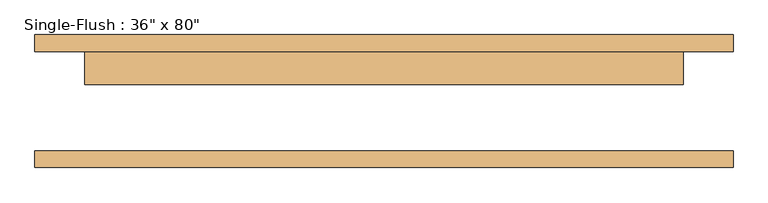
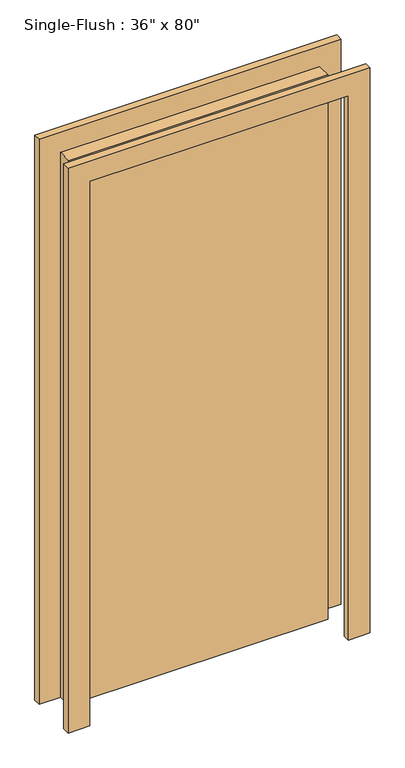
"""IFC4 building model written with IfcOpenShell, lengths in millimetres: door geometry."""

import ifcopenshell
import ifcopenshell.guid

model = None  # the IFC model being written
_history = None  # IfcOwnerHistory: only IFC2X3 demands one
_inside = {}  # id of a spatial element -> (the spatial element, [elements in it])
_under = {}  # id of a project, library or spatial element -> (it, [spatial elements below it])
_declared = {}  # id of a project -> (the project, [libraries it declares])
_typed = {}  # id of a type object -> (the type object, [elements of that type])
_made_of = {}  # id of a material, layer set ... -> (it, [elements and type objects made of it])


def new_model(schema):
    """Start an empty IFC model of exactly this schema.

    Asked for "IFC4X3", IfcOpenShell would pick the latest addendum, in which some entities
    have other attributes; the version numbers below select the first issue.
    IFC2X3 requires an IfcOwnerHistory on every rooted entity: one is made here for all.
    """
    global model, _history
    if schema == "IFC4X3":
        model = ifcopenshell.file(schema_version=(4, 3, 0, 0))
    else:
        model = ifcopenshell.file(schema=schema)
    _inside.clear()
    _under.clear()
    _declared.clear()
    _typed.clear()
    _made_of.clear()
    _history = None
    if model.schema == "IFC2X3":
        org = make("IfcOrganization", Name="unknown")
        user = make(
            "IfcPersonAndOrganization",
            ThePerson=make("IfcPerson", FamilyName="unknown"),
            TheOrganization=org,
        )
        app = make(
            "IfcApplication",
            ApplicationDeveloper=org,
            Version="unknown",
            ApplicationFullName="unknown",
            ApplicationIdentifier="unknown",
        )
        _history = make(
            "IfcOwnerHistory",
            OwningUser=user,
            OwningApplication=app,
            ChangeAction="ADDED",
            CreationDate=0,
        )
    return model


def make(cls, **values):
    """One entity of the class cls with the attributes given. An attribute that is None is left unset."""
    return model.create_entity(
        cls, **{name: value for name, value in values.items() if value is not None}
    )


def rooted(cls, **values):
    """An entity with a GlobalId (a new one), such as an element, a storey or a relation."""
    return make(cls, GlobalId=ifcopenshell.guid.new(), OwnerHistory=_history, **values)


def si_unit(unit_type, name, prefix=None):
    """IfcSIUnit, for example si_unit("LENGTHUNIT", "METRE", prefix="MILLI")."""
    return make("IfcSIUnit", UnitType=unit_type, Prefix=prefix, Name=name)


def assignment(units):
    """IfcUnitAssignment: the units of a project."""
    return None if units is None else make("IfcUnitAssignment", Units=units)


def point(xyz):
    """IfcCartesianPoint."""
    return None if xyz is None else make("IfcCartesianPoint", Coordinates=xyz)


def direction(xyz):
    """IfcDirection."""
    return None if xyz is None else make("IfcDirection", DirectionRatios=xyz)


def frame(location, z_axis=None, x_axis=None):
    """IfcAxis2Placement3D, a coordinate frame: its origin and axes. An axis left out is left unset."""
    return make(
        "IfcAxis2Placement3D",
        Location=point(location),
        Axis=direction(z_axis),
        RefDirection=direction(x_axis),
    )


def origin():
    """The frame at (0, 0, 0) with its axes left unset."""
    return frame((0.0, 0.0, 0.0))


def origin_with_axes():
    """The frame at (0, 0, 0) with the z axis (0, 0, 1) and the x axis (1, 0, 0) written out."""
    return frame((0.0, 0.0, 0.0), z_axis=(0.0, 0.0, 1.0), x_axis=(1.0, 0.0, 0.0))


def place(relative_to, where):
    """IfcLocalPlacement: puts the frame where relative to a parent placement (None: the world)."""
    return make(
        "IfcLocalPlacement", PlacementRelTo=relative_to, RelativePlacement=where
    )


def context(
    kind, dimensions, precision=None, world=None, true_north=None, identifier=None
):
    """IfcGeometricRepresentationContext, for example the 3D "Model" context."""
    return make(
        "IfcGeometricRepresentationContext",
        ContextIdentifier=identifier,
        ContextType=kind,
        CoordinateSpaceDimension=dimensions,
        Precision=precision,
        WorldCoordinateSystem=world,
        TrueNorth=true_north,
    )


def project(units=None, contexts=None):
    """IfcProject with its units and contexts."""
    return rooted(
        "IfcProject",
        Name="project",
        RepresentationContexts=contexts,
        UnitsInContext=assignment(units),
    )


def spatial(cls, under=None, at=None, **own):
    """A site, building, storey or space (cls), placed at a placement, below another one or the project."""
    s = rooted(cls, ObjectPlacement=at, **own)
    if under is not None:
        _under.setdefault(under.id(), (under, []))[1].append(s)
    return s


def polyline(points):
    """IfcPolyline through the points."""
    return make("IfcPolyline", Points=[point(p) for p in points])


def outline(outer, holes=None, kind="AREA"):
    """IfcArbitraryClosedProfileDef: a profile drawn as a closed curve; with holes, ...WithVoids."""
    if holes is None:
        return make("IfcArbitraryClosedProfileDef", ProfileType=kind, OuterCurve=outer)
    return make(
        "IfcArbitraryProfileDefWithVoids",
        ProfileType=kind,
        OuterCurve=outer,
        InnerCurves=holes,
    )


def extrude(swept, where, along, depth):
    """IfcExtrudedAreaSolid: the profile swept, set in the frame where, extruded along a direction by depth."""
    return make(
        "IfcExtrudedAreaSolid",
        SweptArea=swept,
        Position=where,
        ExtrudedDirection=direction(along),
        Depth=depth,
    )


def shape(context_of_items, identifier, shape_type, items):
    """IfcShapeRepresentation: the items that make up one representation, for example the "Body"."""
    return make(
        "IfcShapeRepresentation",
        ContextOfItems=context_of_items,
        RepresentationIdentifier=identifier,
        RepresentationType=shape_type,
        Items=items,
    )


def source(mapping_origin, context_of_items, identifier, shape_type, items):
    """IfcRepresentationMap: a shape defined once, which mapped items show again and again."""
    return make(
        "IfcRepresentationMap",
        MappingOrigin=mapping_origin,
        MappedRepresentation=shape(context_of_items, identifier, shape_type, items),
    )


def transform(
    local_origin,
    x_axis=None,
    y_axis=None,
    z_axis=None,
    scale=None,
    scale2=None,
    scale3=None,
    uniform=True,
):
    """IfcCartesianTransformationOperator3D, or its non-uniform kind. x_axis, y_axis, z_axis: its Axis1, 2, 3."""
    if uniform:
        return make(
            "IfcCartesianTransformationOperator3D",
            Axis1=direction(x_axis),
            Axis2=direction(y_axis),
            LocalOrigin=point(local_origin),
            Scale=scale,
            Axis3=direction(z_axis),
        )
    return make(
        "IfcCartesianTransformationOperator3DnonUniform",
        Axis1=direction(x_axis),
        Axis2=direction(y_axis),
        LocalOrigin=point(local_origin),
        Scale=scale,
        Axis3=direction(z_axis),
        Scale2=scale2,
        Scale3=scale3,
    )


def mapped(mapping_source, mapping_target):
    """IfcMappedItem: shows the shape of a source again, moved by a transform."""
    return make(
        "IfcMappedItem", MappingSource=mapping_source, MappingTarget=mapping_target
    )


def made_of(thing, what):
    """Note that an element or type object is made of a material, layer set ...; save() writes the relation."""
    if what is not None:
        _made_of.setdefault(what.id(), (what, []))[1].append(thing)
    return thing


def element(
    cls,
    number,
    at=None,
    inside=None,
    cuts=None,
    type_object=None,
    material=None,
    context=None,
    identifier="Body",
    shape_type=None,
    held_by="IfcProductDefinitionShape",
    body=None,
    shapes=None,
    **own,
):
    """One element of the class cls, such as IfcWall. Its Tag is "e" and its number.

    at: its placement. inside: the storey or other place that contains it. cuts: it is an
    opening in that element (IfcRelVoidsElement). A single representation is given by context,
    identifier, shape_type and body (its items); several are given by shapes. held_by: the class
    of the entity that holds the representations. save() writes the other relations.
    """
    e = rooted(cls, Tag="e%d" % number, ObjectPlacement=at, **own)
    if body is not None:
        shapes = [shape(context, identifier, shape_type, body)]
    if shapes is not None:
        e.Representation = make(held_by, Representations=shapes)
    if inside is not None:
        _inside.setdefault(inside.id(), (inside, []))[1].append(e)
    if cuts is not None:
        rooted(
            "IfcRelVoidsElement", RelatingBuildingElement=cuts, RelatedOpeningElement=e
        )
    if type_object is not None:
        _typed.setdefault(type_object.id(), (type_object, []))[1].append(e)
    return made_of(e, material)


def aggregate(whole, parts):
    """IfcRelAggregates: a whole, such as a stair, and the parts it consists of."""
    return rooted("IfcRelAggregates", RelatingObject=whole, RelatedObjects=parts)


def save(model, path):
    """Write the relations noted so far, then the file.

    IfcRelAggregates (storeys below a building ...), IfcRelContainedInSpatialStructure (elements
    in a storey), IfcRelDefinesByType, IfcRelAssociatesMaterial and IfcRelDeclares: one each for
    every whole, place, type object, material and project.
    """
    for whole, parts in _under.values():
        aggregate(whole, parts)
    for where, things in _inside.values():
        rooted(
            "IfcRelContainedInSpatialStructure",
            RelatedElements=things,
            RelatingStructure=where,
        )
    for kind, things in _typed.values():
        rooted("IfcRelDefinesByType", RelatedObjects=things, RelatingType=kind)
    for what, things in _made_of.values():
        rooted("IfcRelAssociatesMaterial", RelatedObjects=things, RelatingMaterial=what)
    for by, libraries in _declared.values():
        rooted("IfcRelDeclares", RelatingContext=by, RelatedDefinitions=libraries)
    model.write(path)


def door_193fcfdc(model_context):
    return source(origin(), model_context, "Body", "SweptSolid", [
        extrude(outline(polyline([(2108.2, -533.4), (0.0, -533.4), (0.0, -457.2), (2032.0, -457.2), (2032.0, 457.2), (0.0, 457.2), (0.0, 533.4), (2108.2, 533.4), (2108.2, -533.4)])), frame((0.0, 76.2, 0.0), z_axis=(0.0, 1.0, 0.0), x_axis=(0.0, 0.0, 1.0)), (0.0, 0.0, 1.0), 25.4),
        extrude(outline(polyline([(2108.2, 533.4), (2108.2, -533.4), (0.0, -533.4), (0.0, -457.2), (2032.0, -457.2), (2032.0, 457.2), (0.0, 457.2), (0.0, 533.4), (2108.2, 533.4)])), frame((0.0, -101.6, 0.0), z_axis=(0.0, 1.0, 0.0), x_axis=(0.0, 0.0, 1.0)), (0.0, 0.0, 1.0), 25.4),
        extrude(outline(polyline([(457.2, 25.4), (-457.2, 25.4), (-457.2, 76.2), (457.2, 76.2), (457.2, 25.4)])), origin_with_axes(), (0.0, 0.0, 1.0), 2032.0),
    ])


if __name__ == "__main__":
    model = new_model("IFC4")
    model_context = context("Model", 3, world=origin())
    ifc_project = project(units=[si_unit("LENGTHUNIT", "METRE", prefix="MILLI")], contexts=[model_context])
    site = spatial("IfcSite", under=ifc_project)
    building = spatial("IfcBuilding", under=site)
    placement = place(None, origin())
    door_shape = door_193fcfdc(model_context)
    element("IfcDoor", 1, ObjectType="Single-Flush : 36\" x 80\"", at=placement, inside=building, context=model_context, shape_type="MappedRepresentation", body=[
        mapped(door_shape, transform((0.0, 0.0, 0.0), x_axis=(1.0, 0.0, 0.0), y_axis=(0.0, 1.0, 0.0), z_axis=(0.0, 0.0, 1.0))),
    ])
    save(model, "model.ifc")

# Revit data of these elements
# Type "Single-Flush : 36\" x 80\""
#   Type Mark = "6"
#   Assembly Code = "C1020"
#   Thickness = 0' - 2"
#   Height = 6' - 8"
#   Trim Projection Ext = 0' - 1"
#   Trim Projection Int = 0' - 1"
#   Trim Width = 0' - 3"
#   Width = 3' - 0"
#   Door Material = Door - Panel
#   Frame Material = Door - Frame
#   Function = (empty or 0)
#   Wall Closure = (empty or 0)
# Element 1 (IfcDoor, "Single-Flush : 36\" x 80\"")
#   Materials on its faces: "Door - Frame", "Door - Panel"
# Materials
#   "Door - Panel": class "Wood", colour RGB 114 82 51, transparency 0
#   "Door - Frame": class "Miscellaneous", colour RGB 153 76 43, transparency 0
